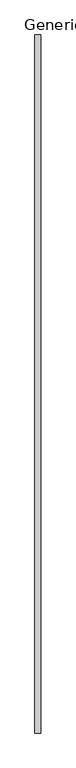
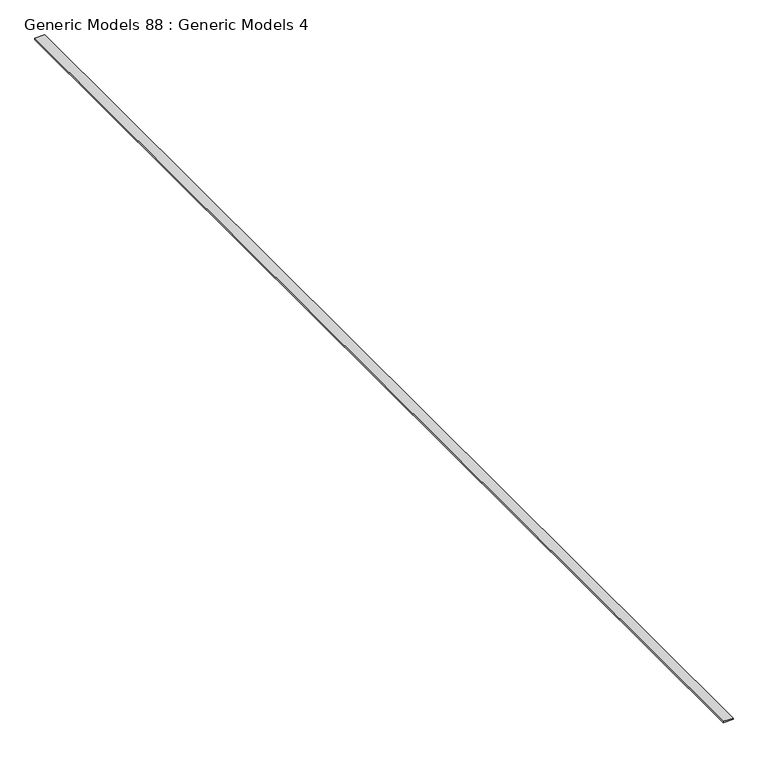
"""IFC4 building model written with IfcOpenShell, lengths in millimetres: proxy geometry, Generic Models 88 : Generic Models 4."""

import ifcopenshell
import ifcopenshell.guid

model = None  # the IFC model being written
_history = None  # IfcOwnerHistory: only IFC2X3 demands one
_inside = {}  # id of a spatial element -> (the spatial element, [elements in it])
_under = {}  # id of a project, library or spatial element -> (it, [spatial elements below it])
_declared = {}  # id of a project -> (the project, [libraries it declares])
_typed = {}  # id of a type object -> (the type object, [elements of that type])
_made_of = {}  # id of a material, layer set ... -> (it, [elements and type objects made of it])


def new_model(schema):
    """Start an empty IFC model of exactly this schema.

    Asked for "IFC4X3", IfcOpenShell would pick the latest addendum, in which some entities
    have other attributes; the version numbers below select the first issue.
    IFC2X3 requires an IfcOwnerHistory on every rooted entity: one is made here for all.
    """
    global model, _history
    if schema == "IFC4X3":
        model = ifcopenshell.file(schema_version=(4, 3, 0, 0))
    else:
        model = ifcopenshell.file(schema=schema)
    _inside.clear()
    _under.clear()
    _declared.clear()
    _typed.clear()
    _made_of.clear()
    _history = None
    if model.schema == "IFC2X3":
        org = make("IfcOrganization", Name="unknown")
        user = make(
            "IfcPersonAndOrganization",
            ThePerson=make("IfcPerson", FamilyName="unknown"),
            TheOrganization=org,
        )
        app = make(
            "IfcApplication",
            ApplicationDeveloper=org,
            Version="unknown",
            ApplicationFullName="unknown",
            ApplicationIdentifier="unknown",
        )
        _history = make(
            "IfcOwnerHistory",
            OwningUser=user,
            OwningApplication=app,
            ChangeAction="ADDED",
            CreationDate=0,
        )
    return model


def make(cls, **values):
    """One entity of the class cls with the attributes given. An attribute that is None is left unset."""
    return model.create_entity(
        cls, **{name: value for name, value in values.items() if value is not None}
    )


def rooted(cls, **values):
    """An entity with a GlobalId (a new one), such as an element, a storey or a relation."""
    return make(cls, GlobalId=ifcopenshell.guid.new(), OwnerHistory=_history, **values)


def si_unit(unit_type, name, prefix=None):
    """IfcSIUnit, for example si_unit("LENGTHUNIT", "METRE", prefix="MILLI")."""
    return make("IfcSIUnit", UnitType=unit_type, Prefix=prefix, Name=name)


def assignment(units):
    """IfcUnitAssignment: the units of a project."""
    return None if units is None else make("IfcUnitAssignment", Units=units)


def point(xyz):
    """IfcCartesianPoint."""
    return None if xyz is None else make("IfcCartesianPoint", Coordinates=xyz)


def direction(xyz):
    """IfcDirection."""
    return None if xyz is None else make("IfcDirection", DirectionRatios=xyz)


def frame(location, z_axis=None, x_axis=None):
    """IfcAxis2Placement3D, a coordinate frame: its origin and axes. An axis left out is left unset."""
    return make(
        "IfcAxis2Placement3D",
        Location=point(location),
        Axis=direction(z_axis),
        RefDirection=direction(x_axis),
    )


def origin():
    """The frame at (0, 0, 0) with its axes left unset."""
    return frame((0.0, 0.0, 0.0))


def place(relative_to, where):
    """IfcLocalPlacement: puts the frame where relative to a parent placement (None: the world)."""
    return make(
        "IfcLocalPlacement", PlacementRelTo=relative_to, RelativePlacement=where
    )


def context(
    kind, dimensions, precision=None, world=None, true_north=None, identifier=None
):
    """IfcGeometricRepresentationContext, for example the 3D "Model" context."""
    return make(
        "IfcGeometricRepresentationContext",
        ContextIdentifier=identifier,
        ContextType=kind,
        CoordinateSpaceDimension=dimensions,
        Precision=precision,
        WorldCoordinateSystem=world,
        TrueNorth=true_north,
    )


def project(units=None, contexts=None):
    """IfcProject with its units and contexts."""
    return rooted(
        "IfcProject",
        Name="project",
        RepresentationContexts=contexts,
        UnitsInContext=assignment(units),
    )


def spatial(cls, under=None, at=None, **own):
    """A site, building, storey or space (cls), placed at a placement, below another one or the project."""
    s = rooted(cls, ObjectPlacement=at, **own)
    if under is not None:
        _under.setdefault(under.id(), (under, []))[1].append(s)
    return s


def polyline(points):
    """IfcPolyline through the points."""
    return make("IfcPolyline", Points=[point(p) for p in points])


def outline(outer, holes=None, kind="AREA"):
    """IfcArbitraryClosedProfileDef: a profile drawn as a closed curve; with holes, ...WithVoids."""
    if holes is None:
        return make("IfcArbitraryClosedProfileDef", ProfileType=kind, OuterCurve=outer)
    return make(
        "IfcArbitraryProfileDefWithVoids",
        ProfileType=kind,
        OuterCurve=outer,
        InnerCurves=holes,
    )


def extrude(swept, where, along, depth):
    """IfcExtrudedAreaSolid: the profile swept, set in the frame where, extruded along a direction by depth."""
    return make(
        "IfcExtrudedAreaSolid",
        SweptArea=swept,
        Position=where,
        ExtrudedDirection=direction(along),
        Depth=depth,
    )


def shape(context_of_items, identifier, shape_type, items):
    """IfcShapeRepresentation: the items that make up one representation, for example the "Body"."""
    return make(
        "IfcShapeRepresentation",
        ContextOfItems=context_of_items,
        RepresentationIdentifier=identifier,
        RepresentationType=shape_type,
        Items=items,
    )


def source(mapping_origin, context_of_items, identifier, shape_type, items):
    """IfcRepresentationMap: a shape defined once, which mapped items show again and again."""
    return make(
        "IfcRepresentationMap",
        MappingOrigin=mapping_origin,
        MappedRepresentation=shape(context_of_items, identifier, shape_type, items),
    )


def transform(
    local_origin,
    x_axis=None,
    y_axis=None,
    z_axis=None,
    scale=None,
    scale2=None,
    scale3=None,
    uniform=True,
):
    """IfcCartesianTransformationOperator3D, or its non-uniform kind. x_axis, y_axis, z_axis: its Axis1, 2, 3."""
    if uniform:
        return make(
            "IfcCartesianTransformationOperator3D",
            Axis1=direction(x_axis),
            Axis2=direction(y_axis),
            LocalOrigin=point(local_origin),
            Scale=scale,
            Axis3=direction(z_axis),
        )
    return make(
        "IfcCartesianTransformationOperator3DnonUniform",
        Axis1=direction(x_axis),
        Axis2=direction(y_axis),
        LocalOrigin=point(local_origin),
        Scale=scale,
        Axis3=direction(z_axis),
        Scale2=scale2,
        Scale3=scale3,
    )


def mapped(mapping_source, mapping_target):
    """IfcMappedItem: shows the shape of a source again, moved by a transform."""
    return make(
        "IfcMappedItem", MappingSource=mapping_source, MappingTarget=mapping_target
    )


def made_of(thing, what):
    """Note that an element or type object is made of a material, layer set ...; save() writes the relation."""
    if what is not None:
        _made_of.setdefault(what.id(), (what, []))[1].append(thing)
    return thing


def element(
    cls,
    number,
    at=None,
    inside=None,
    cuts=None,
    type_object=None,
    material=None,
    context=None,
    identifier="Body",
    shape_type=None,
    held_by="IfcProductDefinitionShape",
    body=None,
    shapes=None,
    **own,
):
    """One element of the class cls, such as IfcWall. Its Tag is "e" and its number.

    at: its placement. inside: the storey or other place that contains it. cuts: it is an
    opening in that element (IfcRelVoidsElement). A single representation is given by context,
    identifier, shape_type and body (its items); several are given by shapes. held_by: the class
    of the entity that holds the representations. save() writes the other relations.
    """
    e = rooted(cls, Tag="e%d" % number, ObjectPlacement=at, **own)
    if body is not None:
        shapes = [shape(context, identifier, shape_type, body)]
    if shapes is not None:
        e.Representation = make(held_by, Representations=shapes)
    if inside is not None:
        _inside.setdefault(inside.id(), (inside, []))[1].append(e)
    if cuts is not None:
        rooted(
            "IfcRelVoidsElement", RelatingBuildingElement=cuts, RelatedOpeningElement=e
        )
    if type_object is not None:
        _typed.setdefault(type_object.id(), (type_object, []))[1].append(e)
    return made_of(e, material)


def aggregate(whole, parts):
    """IfcRelAggregates: a whole, such as a stair, and the parts it consists of."""
    return rooted("IfcRelAggregates", RelatingObject=whole, RelatedObjects=parts)


def save(model, path):
    """Write the relations noted so far, then the file.

    IfcRelAggregates (storeys below a building ...), IfcRelContainedInSpatialStructure (elements
    in a storey), IfcRelDefinesByType, IfcRelAssociatesMaterial and IfcRelDeclares: one each for
    every whole, place, type object, material and project.
    """
    for whole, parts in _under.values():
        aggregate(whole, parts)
    for where, things in _inside.values():
        rooted(
            "IfcRelContainedInSpatialStructure",
            RelatedElements=things,
            RelatingStructure=where,
        )
    for kind, things in _typed.values():
        rooted("IfcRelDefinesByType", RelatedObjects=things, RelatingType=kind)
    for what, things in _made_of.values():
        rooted("IfcRelAssociatesMaterial", RelatedObjects=things, RelatingMaterial=what)
    for by, libraries in _declared.values():
        rooted("IfcRelDeclares", RelatingContext=by, RelatedDefinitions=libraries)
    model.write(path)


def generic_models_88_generic_models_4_f8f801a1(model_context):
    return source(origin(), model_context, "Body", "SweptSolid", [
        extrude(outline(polyline([(7243.9063704, -6864.9230338), (7087.6963704, -6864.9230338), (7087.6963704, 11778.6769662), (7243.9063704, 11778.6769662), (7243.9063704, -6864.9230338)])), frame((0.0, 0.0, 126304.421), z_axis=(0.0, 0.0, 1.0), x_axis=(1.0, 0.0, 0.0)), (0.0, 0.0, 1.0), 22.225),
    ])


if __name__ == "__main__":
    model = new_model("IFC4")
    model_context = context("Model", 3, world=origin())
    ifc_project = project(units=[si_unit("LENGTHUNIT", "METRE", prefix="MILLI")], contexts=[model_context])
    site = spatial("IfcSite", under=ifc_project)
    building = spatial("IfcBuilding", under=site)
    placement = place(None, origin())
    generic_models_88_generic_models_4_shape = generic_models_88_generic_models_4_f8f801a1(model_context)
    element("IfcBuildingElementProxy", 1, Name="Generic Models 88 : Generic Models 4", ObjectType="Generic Models 88 : Generic Models 4", at=placement, inside=building, context=model_context, shape_type="MappedRepresentation", body=[
        mapped(generic_models_88_generic_models_4_shape, transform((0.0, 0.0, 0.0), x_axis=(1.0, 0.0, 0.0), y_axis=(0.0, 1.0, 0.0), z_axis=(0.0, 0.0, 1.0))),
    ])
    save(model, "model.ifc")

# Revit data of these elements
# Element 1 (IfcBuildingElementProxy, "Generic Models 88 : Generic Models 4")
#   Materials on its faces: "_7/8\" SMOOTH TROWEL EXTERIOR STUCCO (COLOR PER OWNER)"
# Materials
#   "_7/8\" SMOOTH TROWEL EXTERIOR STUCCO (COLOR PER OWNER)": class "Generic", colour RGB 233 233 233, transparency 0, Cost = 0
